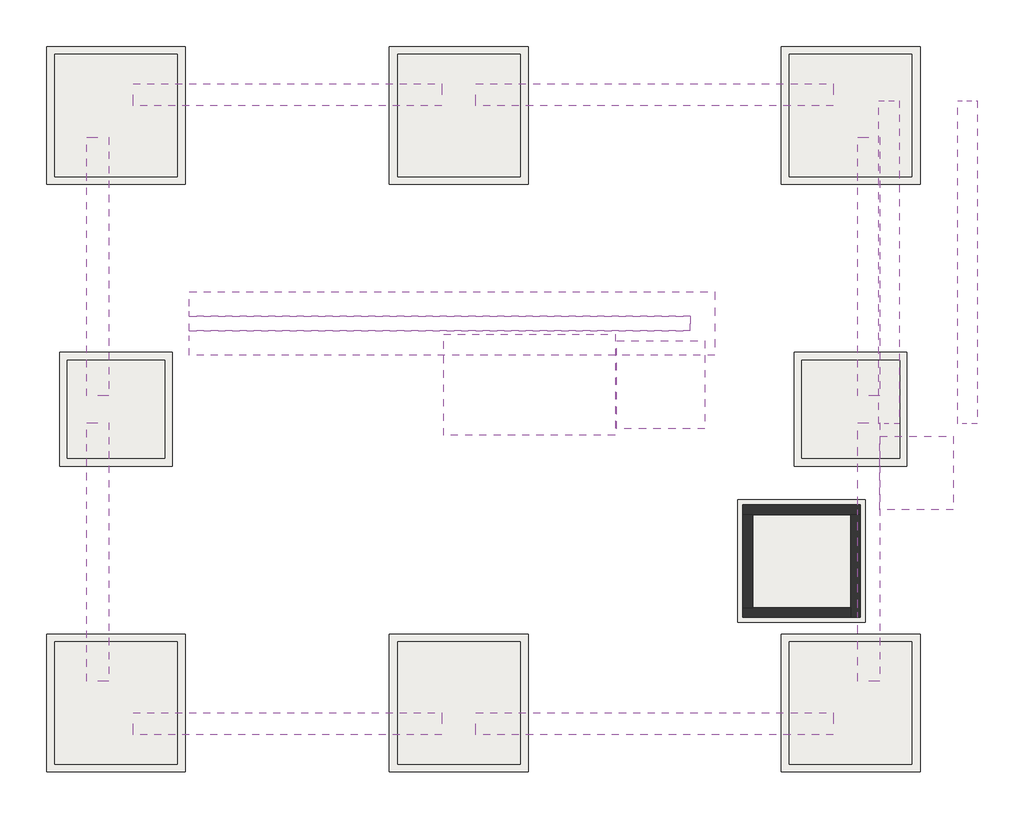
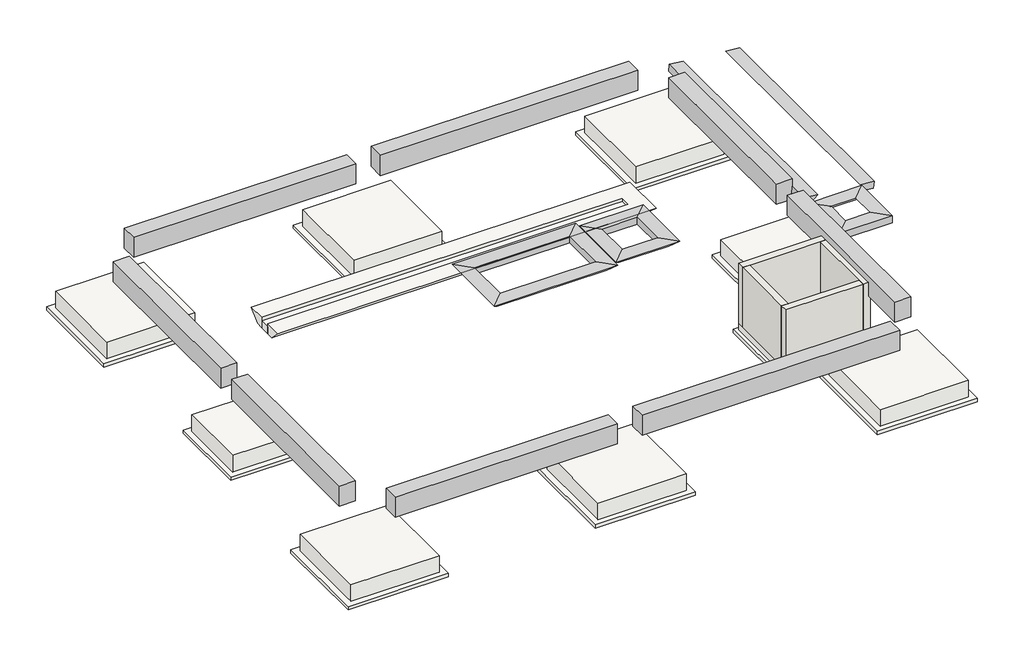
# One storey: 20 slabs, 7 beams, 5 proxies, 4 walls, 1 member.
# Revit data of these elements (continued)
# Project information (continued)
#     93-00152f0a\" ism_id=\"434ac00d-0b75-408a-b526-bf8655b26baf\" /><element revit_id=\"af7cfdda-f71a-4a09-bb03-63e0c16d5d93-00152f0c\" ism_id=\"5e4f7e2a-2154-47cc-93bc-24e7bd197632\" /><element revit_id=\"af7cfdda-f71a-4a09-bb03-63e0c16d5d93-00152f0e\" ism_id=\"f1998cd9-044c-4f7a-99e6-248bc5b45dba\" /><element revit_id=\"af7cfdda-f71a-4a09-bb03-63e0c16d5d93-00152f10\" ism_id=\"6ca0e144-6dd7-4824-b6a4-c3599ffcc64c\" /><element revit_id=\"af7cfdda-f71a-4a09-bb03-63e0c16d5d93-00152f12\" ism_id=\"173f1f07-ca52-4750-b7f6-1ef0180c36ba\" /><element revit_id=\"af7cfdda-f71a-4a09-bb03-63e0c16d5d93-00152f15\" ism_id=\"29a619d1-86ac-46c7-a220-2e78769b313e\" /><element revit_id=\"af7cfdda-f71a-4a09-bb03-63e0c16d5d93-00152f17\" ism_id=\"de21b25d-6b5e-4da6-89ee-8b671f1287ec\" /><element revit_id=\"af7cfdda-f71a-4a09-bb03-63e0c16d5d93-00152f19\" ism_id=\"70cdf538-eeaa-48c4-9315-181e56578638\" /><element revit_id=\"af7cfdda-f71a-4a09-bb03-63e0c16d5d93-00152f1b\" ism_id=\"49734cf8-a963-4163-b104-a25bff74fff0\" /><element revit_id=\"af7cfdda-f71a-4a09-bb03-63e0c16d5d93-00152f1d\" ism_id=\"a5a98e28-e98d-4759-bcab-d40632bfc19f\" /><element revit_id=\"af7cfdda-f71a-4a09-bb03-63e0c16d5d93-00152f1f\" ism_id=\"ab6af08f-90da-4d2f-a66a-db65621b8e94\" /><element revit_id=\"af7cfdda-f71a-4a09-bb03-63e0c16d5d93-00152f21\" ism_id=\"a65b64ab-134d-4223-82b7-5e66d90bc276\" /><element revit_id=\"af7cfdda-f71a-4a09-bb03-63e0c16d5d93-00152f23\" ism_id=\"6a1f317f-8940-4af8-9522-8e6c47c0c3a6\" /><element revit_id=\"af7cfdda-f71a-4a09-bb03-63e0c16d5d93-00152f25\" ism_id=\"880c6aab-7058-4382-9d83-6c759bdcf822\" /><element revit_id=\"af7cfdda-f71a-4a09-bb03-63e0c16d5d93-00152f27\" ism_id=\"555977b1-6494-4ee8-b235-8bae97762787\" /><element revit_id=\"af7cfdda-f71a-4a09-bb03-63e0c16d5d93-00152f29\" ism_id=\"66c9b467-8c65-4f1e-9542-95b43d793e9b\" /><element revit_id=\"af7cfdda-f71a-4a09-bb03-63e0c16d5d93-00152f2b\" ism_id=\"217a9ce2-64ab-4115-836e-06014fa1b21e\" /><element revit_id=\"af7cfdda-f71a-4a09-bb03-63e0c16d5d93-00152f2d\" ism_id=\"f7fc30da-832d-44e7-bab3-dd115d25639e\" /><element revit_id=\"af7cfdda-f71a-4a09-bb03-63e0c16d5d93-00152f2f\" ism_id=\"715eb46c-1b8d-4226-a7c6-6c6c165bf34d\" /><element revit_id=\"af7cfdda-f71a-4a09-bb03-63e0c16d5d93-00152f31\" ism_id=\"ef53c2b2-6fcf-42d2-96ea-f30a899bf64f\" /><element revit_id=\"af7cfdda-f71a-4a09-bb03-63e0c16d5d93-00152f34\" ism_id=\"1aefa093-18ee-4a97-8178-1b1fb4b7aceb\" /><element revit_id=\"af7cfdda-f71a-4a09-bb03-63e0c16d5d93-00152f38\" ism_id=\"262f02a9-64ca-487b-befd-4b58d44dffa7\" /><element revit_id=\"af7cfdda-f71a-4a09-bb03-63e0c16d5d93-00152f3b\" ism_id=\"6f2442a8-c4c0-4b53-9d7f-7059d6ededd2\" /><element revit_id=\"af7cfdda-f71a-4a09-bb03-63e0c16d5d93-00152f3e\" ism_id=\"dd838df4-69c7-406c-93e1-418c01f5734f\" /><element revit_id=\"af7cfdda-f71a-4a09-bb03-63e0c16d5d93-00152f40\" ism_id=\"9dec5077-28a7-4c32-95d2-08813de6a916\" /><element revit_id=\"af7cfdda-f71a-4a09-bb03-63e0c16d5d93-00152f42\" ism_id=\"9370ae5f-9277-4bb3-917b-cb3f318800a8\" /><element revit_id=\"af7cfdda-f71a-4a09-bb03-63e0c16d5d93-00152f44\" ism_id=\"0f3f2c81-58b4-4698-b1be-75061a4a2ae1\" /><element revit_id=\"af7cfdda-f71a-4a09-bb03-63e0c16d5d93-00152f46\" ism_id=\"95dca10f-6510-4ae7-a23e-7a1fd6939662\" /><element revit_id=\"af7cfdda-f71a-4a09-bb03-63e0c16d5d93-00152f49\" ism_id=\"83bad907-6a1c-4702-9990-a1a9c13d0160\" /><element revit_id=\"af7cfdda-f71a-4a09-bb03-63e0c16d5d93-00152f4d\" ism_id=\"7dba72dc-0de8-457c-8d3c-9c80941133ff\" /><element revit_id=\"af7cfdda-f71a-4a09-bb03-63e0c16d5d93-00152f51\" ism_id=\"a6cf3de2-949b-45b4-8029-061e06e5ab91\" /><element revit_id=\"af7cfdda-f71a-4a09-bb03-63e0c16d5d93-00152f54\" ism_id=\"77af5754-dd62-4c90-accb-d0b9405b5baf\" /><element revit_id=\"af7cfdda-f71a-4a09-bb03-63e0c16d5d93-00152f56\" ism_id=\"6461cb37-823d-49bb-bea2-3dbd4db85a81\" /><element revit_id=\"af7cfdda-f71a-4a09-bb03-63e0c16d5d93-00152f59\" ism_id=\"e2f2909f-27bc-426e-b2db-27b1217d3560\" /><element revit_id=\"af7cfdda-f71a-4a09-bb03-63e0c16d5d93-00152f5b\" ism_id=\"46c410de-fc65-4593-ae24-da1a154b45fb\" /><element revit_id=\"af7cfdda-f71a-4a09-bb03-63e0c16d5d93-00152f5d\" ism_id=\"d7d73cf7-a31f-421c-bc39-3ba338a334b1\" /><element revit_id=\"af7cfdda-f71a-4a09-bb03-63e0c16d5d93-00152f61\" ism_id=\"6bd81f7b-5fd8-4f19-ad3a-4e009274854c\" /><element revit_id=\"af7cfdda-f71a-4a09-bb03-63e0c16d5d93-00152f64\" ism_id=\"f25b9af0-504f-4aaf-a359-d2bc9d32b683\" /><element revit_id=\"af7cfdda-f71a-4a09-bb03-63e0c16d5d93-00152f66\" ism_id=\"f143dcd3-1cc7-47ae-b4ed-c960a7d1349c\" /><element revit_id=\"af7cfdda-f71a-4a09-bb03-63e0c16d5d93-00152f68\" ism_id=\"296e8d7f-a89b-405a-b793-fc1ea4b11be5\" /><element revit_id=\"af7cfdda-f71a-4a09-bb03-63e0c16d5d93-00152f6b\" ism_id=\"48b24488-3184-439c-b285-73e81edfef17\" /><element revit_id=\"af7cfdda-f71a-4a09-bb03-63e0c16d5d93-00152f6e\" ism_id=\"0db0ccd4-631c-4972-aad8-2fd483c55629\" /><element revit_id=\"af7cfdda-f71a-4a09-bb03-63e0c16d5d93-00152f71\" ism_id=\"ee51bd40-01d8-4a48-92c6-90509a96cad2\" /><element revit_id=\"af7cfdda-f71a-4a09-bb03-63e0c16d5d93-00152f73\" ism_id=\"e5c66ce6-ca9d-4591-9d75-5348307a88bc\" /><element revit_id=\"af7cfdda-f71a-4a09-bb03-63e0c16d5d93-00152f75\" ism_id=\"892d82ae-6f73-4af5-8575-78955f2b6c3b\" /><element revit_id=\"af7cfdda-f71a-4a09-bb03-63e0c16d5d93-00152f78\" ism_id=\"cb5b2a2e-5551-4b87-9d0b-6382c09e6ce2\" /><element revit_id=\"af7cfdda-f71a-4a09-bb03-63e0c16d5d93-00152f7c\" ism_id=\"1177c4ab-d04b-426b-80ba-afa1f1403e20\" /><element revit_id=\"af7cfdda-f71a-4a09-bb03-63e0c16d5d93-00152f7f\" ism_id=\"235d8a18-f10a-44ad-8945-ebb2f02646fa\" /><element revit_id=\"af7cfdda-f71a-4a09-bb03-63e0c16d5d93-00152f83\" ism_id=\"6127db9d-7d4b-44c8-806c-e4f7d278db0c\" /><element revit_id=\"af7cfdda-f71a-4a09-bb03-63e0c16d5d93-00152f86\" ism_id=\"85d79da8-d317-4e5b-88a2-88d20cb73d7d\" /><element revit_id=\"af7cfdda-f71a-4a09-bb03-63e0c16d5d93-00152f89\" ism_id=\"f4105a19-7c5e-4970-9446-50e578b67af2\" /><element revit_id=\"af7cfdda-f71a-4a09-bb03-63e0c16d5d93-00152f8b\" ism_id=\"ab299061-87b1-4edc-8a5c-c55542368f39\" /><element revit_id=\"af7cfdda-f71a-4a09-bb03-63e0c16d5d93-00152f8d\" ism_id=\"43097401-25be-48d4-a7ba-f3c37c1b84e9\" /><element revit_id=\"af7cfdda-f71a-4a09-bb03-63e0c16d5d93-00152f8f\" ism_id=\"fd9214b7-59e9-4736-b544-a37d4c180e24\" /><element revit_id=\"af7cfdda-f71a-4a09-bb03-63e0c16d5d93-00152f91\" ism_id=\"b83d1d95-2d97-4532-8a94-368577601c17\" /><element revit_id=\"af7cfdda-f71a-4a09-bb03-63e0c16d5d93-00152f94\" ism_id=\"9bd5e620-e2eb-4ede-9a8b-b0183e171248\" /><element revit_id=\"af7cfdda-f71a-4a09-bb03-63e0c16d5d93-00152f97\" ism_id=\"d6f9d903-1605-43dc-872c-2f9de6642af6\" /><element revit_id=\"af7cfdda-f71a-4a09-bb03-63e0c16d5d93-00152f99\" ism_id=\"7c236b12-3da8-4ae0-bc99-2aa089118476\" /><element revit_id=\"af7cfdda-f71a-4a09-bb03-63e0c16d5d93-00152f9b\" ism_id=\"2b88d03d-aeef-4f51-b98c-562513d6f6da\" /><element revit_id=\"af7cfdda-f71a-4a09-bb03-63e0c16d5d93-00152f9d\" ism_id=\"6639b07f-6759-4580-bc0a-91cdbc82216d\" /><element revit_id=\"af7cfdda-f71a-4a09-bb03-63e0c16d5d93-00152f9f\" ism_id=\"d17e7cf5-d760-4c38-8bb0-8a57fe45e3ad\" /><element revit_id=\"af7cfdda-f71a-4a09-bb03-63e0c16d5d93-00152fa2\" ism_id=\"6dbdf2a2-22ac-4132-a9ae-8992fe15b0d7\" /><element revit_id=\"af7cfdda-f71a-4a09-bb03-63e0c16d5d93-00152fa4\" ism_id=\"663381be-9f3f-499f-b7c1-64170401ecb3\" /><element revit_id=\"af7cfdda-f71a-4a09-bb03-63e0c16d5d93-00152fa6\" ism_id=\"5ba3ff14-3d24-47a8-9418-aecce16bd943\" /><element revit_id=\"af7cfdda-f71a-4a09-bb03-63e0c16d5d93-00152fa8\" ism_id=\"8f845e6a-1432-4c61-8362-e12c105320fb\" /><element revit_id=\"af7cfdda-f71a-4a09-bb03-63e0c16d5d93-00152faa\" ism_id=\"263897bf-02c2-4ed7-8e3f-2020d545125e\" /><element revit_id=\"af7cfdda-f71a-4a09-bb03-63e0c16d5d93-00152fac\" ism_id=\"f1241312-d990-4c87-92ff-afc1975a3d67\" /><element revit_id=\"af7cfdda-f71a-4a09-bb03-63e0c16d5d93-00152fae\" ism_id=\"5740cb23-0cbc-47ce-acea-31b5a043bf0c\" /><element revit_id=\"af7cfdda-f71a-4a09-bb03-63e0c16d5d93-00152fb0\" ism_id=\"7aeaeafb-f9bc-4bee-b237-caade22069b8\" /><element revit_id=\"af7cfdda-f71a-4a09-bb03-63e0c16d5d93-00152fb3\" ism_id=\"90084dda-e197-4e46-8e5b-4f629a594830\" /><element revit_id=\"af7cfdda-f71a-4a09-bb03-63e0c16d5d93-00152fb5\" ism_id=\"2c392f12-2b50-4bd2-8c41-ef64640e587b\" /><element revit_id=\"af7cfdda-f71a-4a09-bb03-63e0c16d5d93-00152fb7\" ism_id=\"d25284c0-6931-4cbb-8ed3-63397f6a5616\" /><element revit_id=\"af7cfdda-f71a-4a09-bb03-63e0c16d5d93-00152fb9\" ism_id=\"32799d39-e9bc-468c-ac64-a3f2c8e075af\" /><element revit_id=\"af7cfdda-f71a-4a09-bb03-63e0c16d5d93-00152fbb\" ism_id=\"61a092b8-d924-4e61-a1ef-adc051541aaf\" /><element revit_id=\"af7cfdda-f71a-4a09-bb03-63e0c16d5d93-00152fbe\" ism_id=\"ae89ad42-0006-42ee-9328-01a896002b7a\" /><element revit_id=\"af7cfdda-f71a-4a09-bb03-63e0c16d5d93-00152fc0\" ism_id=\"7b4d47fd-5fcd-4692-9b39-36bb95372647\" /><element revit_id=\"af7cfdda-f71a-4a09-bb03-63e0c16d5d93-00152fc2\" ism_id=\"150f022d-eb78-47d8-8d70-c7ea5433f366\" /><element revit_id=\"af7cfdda-f71a-4a09-bb03-63e0c16d5d93-00152fc4\" ism_id=\"6780451e-52c6-4962-8bb4-f1fd57bf7865\" /><element revit_id=\"af7cfdda-f71a-4a09-bb03-63e0c16d5d93-00152fc6\" ism_id=\"b3896748-2d7c-424b-ae81-8b769d840fbc\" /><element revit_id=\"af7cfdda-f71a-4a09-bb03-63e0c16d5d93-00152fc9\" ism_id=\"0c64c745-ce95-4f37-8a9d-d07fd5d17ecb\" /><element revit_id=\"af7cfdda-f71a-4a09-bb03-63e0c16d5d93-00152fcc\" ism_id=\"dc23390d-d501-4d7e-9369-f7793a7306a7\" /><element revit_id=\"af7cfdda-f71a-4a09-bb03-63e0c16d5d93-00152fcf\" ism_id=\"a2d2dfc7-08e7-459b-9de9-2d46c1b9d65d\" /><element revit_id=\"af7cfdda-f71a-4a09-bb03-63e0c16d5d93-00152fd2\" ism_id=\"0357c393-c221-46b8-a525-7eece05024d5\" /><element revit_id=\"af7cfdda-f71a-4a09-bb03-63e0c16d5d93-00152fd4\" ism_id=\"7514ec1a-cc54-428f-bbfe-53465c7b9971\" /><element revit_id=\"af7cfdda-f71a-4a09-bb03-63e0c16d5d93-00152fd7\" ism_id=\"f5e61f1a-565d-4eed-b8cc-74798bf49f83\" /><element revit_id=\"af7cfdda-f71a-4a09-bb03-63e0c16d5d93-00152fd9\" ism_id=\"7d7031a0-6061-49e6-8bb3-df1503ddb602\" /><element revit_id=\"af7cfdda-f71a-4a09-bb03-63e0c16d5d93-00152fdb\" ism_id=\"0d733cbc-e2dd-44ec-a5f3-da43d2d7ec46\" /><element revit_id=\"af7cfdda-f71a-4a09-bb03-63e0c16d5d93-00152fdd\" ism_id=\"21cbc8e9-c640-4a2e-8958-1d3b7a784879\" /><element revit_id=\"af7cfdda-f71a-4a09-bb03-63e0c16d5d93-00152fdf\" ism_id=\"fac86bbb-1d81-4320-81cd-30997be31eb4\" /><element revit_id=\"af7cfdda-f71a-4a09-bb03-63e0c16d5d93-00152fe1\" ism_id=\"ebc7c696-170e-4ba4-8599-103279d331b8\" /><element revit_id=\"af7cfdda-f71a-4a09-bb03-63e0c16d5d93-00152fe3\" ism_id=\"91dec439-7fd8-4259-bbce-df46237765e2\" /><element revit_id=\"af7cfdda-f71a-4a09-bb03-63e0c16d5d93-00152fe5\" ism_id=\"6227503a-c521-4b5a-b5c3-b9e2ea2b5c81\" /><element revit_id=\"af7cfdda-f71a-4a09-bb03-63e0c16d5d93-00152fe7\" ism_id=\"e6e91966-53ab-4536-84a0-3f6e5a22fbeb\" /><element revit_id=\"af7cfdda-f71a-4a09-bb03-63e0c16d5d93-00152fe9\" ism_id=\"fb3387b3-301c-40a5-8217-97be67c50843\" /><element revit_id=\"af7cfdda-f71a-4a09-bb03-63e0c16d5d93-00152feb\" ism_id=\"37825fc8-0fe2-440e-933a-1453c922c9d9\" /><element revit_id=\"af7cfdda-f71a-4a09-bb03-63e0c16d5d93-00152fed\" ism_id=\"06b175df-5526-4920-a3d6-7f2ff872756e\" /><element revit_id=\"af7cfdda-f71a-4a09-bb03-63e0c16d5d93-00152fef\" ism_id=\"a8fbce7a-6989-46e5-9bc5-c497d4a295c9\" /><element revit_id=\"af7cfdda-f71a-4a09-bb03-63e0c16d5d93-00152ff1\" ism_id=\"cf8ccf89-d0da-4b4e-93d8-85d639853d5e\" /><element revit_id=\"af7cfdda-f71a-4a09-bb03-63e0c16d5d93-00152ff3\" ism_id=\"1b85e87c-6c2a-4057-8491-40e4237cd0e6\" /><element revit_id=\"af7cfdda-f71a-4a09-bb03-63e0c16d5d93-00152ff5\" ism_id=\"69be497f-343c-4d38-9ea0-e959474332f8\" /><element revit_id=\"af7cfdda-f71a-4a09-bb03-63e0c16d5d93-00152ff7\" ism_id=\"72738956-f87a-41b4-a019-35adc3bff764\" /><element revit_id=\"af7cfdda-f71a-4a09-bb03-63e0c16d5d93-00152ff9\" ism_id=\"f127b15c-142d-4b57-83a6-5b76ac4cde6e\" /><element revit_id=
#     \"af7cfdda-f71a-4a09-bb03-63e0c16d5d93-00152ffb\" ism_id=\"3a38a709-bfa8-404e-b889-5af5e78ea0bf\" /><element revit_id=\"af7cfdda-f71a-4a09-bb03-63e0c16d5d93-00152ffe\" ism_id=\"bebf0363-7e59-4a43-8f5b-502fcc4a338d\" /><element revit_id=\"af7cfdda-f71a-4a09-bb03-63e0c16d5d93-00153000\" ism_id=\"157fe154-0d28-4e8c-a143-e2896867fd28\" /><element revit_id=\"af7cfdda-f71a-4a09-bb03-63e0c16d5d93-00153002\" ism_id=\"1bf52bf8-7327-4d55-b5cd-bf7c9bf89688\" /><element revit_id=\"af7cfdda-f71a-4a09-bb03-63e0c16d5d93-00153005\" ism_id=\"7a0025bf-d54b-4614-9002-7bd4a82da90e\" /><element revit_id=\"af7cfdda-f71a-4a09-bb03-63e0c16d5d93-00153008\" ism_id=\"cad53638-8c8f-4a89-ab6f-d8a32131833b\" /><element revit_id=\"af7cfdda-f71a-4a09-bb03-63e0c16d5d93-0015300a\" ism_id=\"05672ccd-1a96-434c-8da1-7a706b3561f7\" /><element revit_id=\"af7cfdda-f71a-4a09-bb03-63e0c16d5d93-0015300c\" ism_id=\"bb809016-b2bb-4157-847e-1cca3692ba19\" /><element revit_id=\"af7cfdda-f71a-4a09-bb03-63e0c16d5d93-0015300f\" ism_id=\"720ed192-8aa7-46fd-9f7a-15d64351767c\" /><element revit_id=\"af7cfdda-f71a-4a09-bb03-63e0c16d5d93-00153011\" ism_id=\"9a47cdb9-976d-41f3-a5c3-5a7516a7763c\" /><element revit_id=\"af7cfdda-f71a-4a09-bb03-63e0c16d5d93-00153013\" ism_id=\"aba01787-c82b-453e-8db2-70277a34d5ad\" /><element revit_id=\"af7cfdda-f71a-4a09-bb03-63e0c16d5d93-00153015\" ism_id=\"f6b882e3-d64a-44b1-878c-9c00ee1fde86\" /><element revit_id=\"af7cfdda-f71a-4a09-bb03-63e0c16d5d93-00153017\" ism_id=\"95108815-490a-427a-aec1-8fcefc57c858\" /><element revit_id=\"af7cfdda-f71a-4a09-bb03-63e0c16d5d93-00153019\" ism_id=\"8fe55cf1-56b4-4a62-948a-d7f0c95bd04b\" /><element revit_id=\"af7cfdda-f71a-4a09-bb03-63e0c16d5d93-0015301b\" ism_id=\"b889bf8b-3bdd-410a-b11b-9ca69449d470\" /><element revit_id=\"af7cfdda-f71a-4a09-bb03-63e0c16d5d93-0015301d\" ism_id=\"ef8604de-de5b-45ec-9158-0b702e6ef713\" /><element revit_id=\"af7cfdda-f71a-4a09-bb03-63e0c16d5d93-0015301f\" ism_id=\"40ee286a-4bc9-4d4f-ba6d-fe1ac9da03cf\" /><element revit_id=\"af7cfdda-f71a-4a09-bb03-63e0c16d5d93-00153021\" ism_id=\"cc903f39-6bdf-4081-a56c-883169221735\" /><element revit_id=\"af7cfdda-f71a-4a09-bb03-63e0c16d5d93-00153023\" ism_id=\"0af04955-dcb6-4295-b3d4-7c432a233062\" /><element revit_id=\"af7cfdda-f71a-4a09-bb03-63e0c16d5d93-00153025\" ism_id=\"75a51549-6a04-4399-b818-f170a8c10286\" /><element revit_id=\"af7cfdda-f71a-4a09-bb03-63e0c16d5d93-00153027\" ism_id=\"7e183794-5c66-46bc-97f5-2df209b3286d\" /><element revit_id=\"af7cfdda-f71a-4a09-bb03-63e0c16d5d93-00153029\" ism_id=\"ed4a7448-29b0-44e3-8b6f-7310f83440ab\" /><element revit_id=\"af7cfdda-f71a-4a09-bb03-63e0c16d5d93-0015302b\" ism_id=\"fdb5eb17-b94e-40c1-b703-3ecb5e4efee4\" /><element revit_id=\"af7cfdda-f71a-4a09-bb03-63e0c16d5d93-0015302d\" ism_id=\"779397c1-65b7-447f-a72e-2a09308021ea\" /><element revit_id=\"af7cfdda-f71a-4a09-bb03-63e0c16d5d93-0015302f\" ism_id=\"7b409707-86c5-44e2-919e-92ad5bb9eb8b\" /><element revit_id=\"af7cfdda-f71a-4a09-bb03-63e0c16d5d93-00153031\" ism_id=\"d337c78b-590d-406c-bf20-6a3558821db1\" /><element revit_id=\"af7cfdda-f71a-4a09-bb03-63e0c16d5d93-00153033\" ism_id=\"c27f5f6d-8445-4415-853d-d316787bea6e\" /><element revit_id=\"af7cfdda-f71a-4a09-bb03-63e0c16d5d93-00153035\" ism_id=\"76036a55-3bab-417a-ba41-ec1335e2e2a7\" /><element revit_id=\"af7cfdda-f71a-4a09-bb03-63e0c16d5d93-00153037\" ism_id=\"24be638c-ff89-4616-8974-5b79c81e6e56\" /><element revit_id=\"af7cfdda-f71a-4a09-bb03-63e0c16d5d93-00153039\" ism_id=\"015f9f2c-2353-4795-b891-e4ee986f25f7\" /><element revit_id=\"af7cfdda-f71a-4a09-bb03-63e0c16d5d93-0015303b\" ism_id=\"91f8ddfb-c5b9-4f33-b141-a6edfbccf098\" /><element revit_id=\"af7cfdda-f71a-4a09-bb03-63e0c16d5d93-0015303d\" ism_id=\"78540364-1ba5-4f0c-95fb-ba8631e32695\" /><element revit_id=\"af7cfdda-f71a-4a09-bb03-63e0c16d5d93-0015303f\" ism_id=\"9d53e406-367b-4e3e-b5e8-d421731e1aab\" /><element revit_id=\"af7cfdda-f71a-4a09-bb03-63e0c16d5d93-00153041\" ism_id=\"24aa6051-1a20-4f08-8962-6f6f9ff4dc98\" /><element revit_id=\"af7cfdda-f71a-4a09-bb03-63e0c16d5d93-00153043\" ism_id=\"572a4144-5250-4962-a1b9-09502cda2774\" /><element revit_id=\"af7cfdda-f71a-4a09-bb03-63e0c16d5d93-00153045\" ism_id=\"1f486980-0be9-4aad-b32e-0608218bf68e\" /><element revit_id=\"af7cfdda-f71a-4a09-bb03-63e0c16d5d93-00153047\" ism_id=\"588ed856-d113-4521-b97c-a4d7ac7ba406\" /><element revit_id=\"af7cfdda-f71a-4a09-bb03-63e0c16d5d93-00153049\" ism_id=\"741942b7-995d-48cb-8401-4faec8ef8d15\" /><element revit_id=\"af7cfdda-f71a-4a09-bb03-63e0c16d5d93-0015304b\" ism_id=\"85254c30-08c9-46e3-acd6-6b5131f485ce\" /><element revit_id=\"af7cfdda-f71a-4a09-bb03-63e0c16d5d93-0015304e\" ism_id=\"2d57d6c0-67d8-48bd-b16f-8ef7edb485b1\" /><element revit_id=\"af7cfdda-f71a-4a09-bb03-63e0c16d5d93-00153050\" ism_id=\"57b4caff-473e-4ebc-b42c-d73ce4ca67d8\" /><element revit_id=\"af7cfdda-f71a-4a09-bb03-63e0c16d5d93-00153052\" ism_id=\"1adae240-a487-478c-a898-61bee40e7415\" /><element revit_id=\"af7cfdda-f71a-4a09-bb03-63e0c16d5d93-00153054\" ism_id=\"62613b5f-092e-4f63-86ac-d3e070a85bc5\" /><element revit_id=\"af7cfdda-f71a-4a09-bb03-63e0c16d5d93-00153056\" ism_id=\"6aecb1de-b991-4eed-80ad-e1b9ccc03a87\" /><element revit_id=\"af7cfdda-f71a-4a09-bb03-63e0c16d5d93-00153058\" ism_id=\"ecab5d8d-84d0-44a4-9549-bca959ac514b\" /><element revit_id=\"af7cfdda-f71a-4a09-bb03-63e0c16d5d93-0015305a\" ism_id=\"589f44ad-061b-46bc-91bd-bf9b1e708415\" /><element revit_id=\"af7cfdda-f71a-4a09-bb03-63e0c16d5d93-0015305c\" ism_id=\"bfa24af8-499f-45ff-9e9d-d5cc0761fed6\" /><element revit_id=\"af7cfdda-f71a-4a09-bb03-63e0c16d5d93-0015305e\" ism_id=\"8114f473-ca73-4cc8-b3e2-979f07368f66\" /><element revit_id=\"af7cfdda-f71a-4a09-bb03-63e0c16d5d93-00153060\" ism_id=\"4dde7439-2ac9-412f-a5f5-e9fd0f294ec8\" /><element revit_id=\"af7cfdda-f71a-4a09-bb03-63e0c16d5d93-00153062\" ism_id=\"661cc7d8-fd9c-4505-b43e-241bfd24b2d0\" /><element revit_id=\"af7cfdda-f71a-4a09-bb03-63e0c16d5d93-00153064\" ism_id=\"1e7f186f-1b55-4d4c-bf9f-18595049605e\" /><element revit_id=\"af7cfdda-f71a-4a09-bb03-63e0c16d5d93-00153066\" ism_id=\"ee968183-c9c6-4eab-86cf-0eda12de724b\" /><element revit_id=\"af7cfdda-f71a-4a09-bb03-63e0c16d5d93-00153068\" ism_id=\"5de1f319-cdd1-4b9a-8f8e-b86394effa22\" /><element revit_id=\"af7cfdda-f71a-4a09-bb03-63e0c16d5d93-0015306a\" ism_id=\"fa557a6c-2e39-4481-9eb5-5ede8fd31c49\" /><element revit_id=\"af7cfdda-f71a-4a09-bb03-63e0c16d5d93-0015306c\" ism_id=\"b2710e8e-0f5f-4e74-a366-aef04da22cd3\" /><element revit_id=\"af7cfdda-f71a-4a09-bb03-63e0c16d5d93-0015306e\" ism_id=\"5633c3b7-f903-46ee-b126-8a20a9a62c90\" /><element revit_id=\"af7cfdda-f71a-4a09-bb03-63e0c16d5d93-00153070\" ism_id=\"62796ef8-c4bb-4b9f-bd14-cc7392046eb4\" /><element revit_id=\"af7cfdda-f71a-4a09-bb03-63e0c16d5d93-00153072\" ism_id=\"db898ada-150e-4ff5-a9f8-16e27b46b754\" /><element revit_id=\"af7cfdda-f71a-4a09-bb03-63e0c16d5d93-00153075\" ism_id=\"d3965d2d-e119-4f6b-af8d-52c8a5397d36\" /><element revit_id=\"af7cfdda-f71a-4a09-bb03-63e0c16d5d93-00153077\" ism_id=\"063574e4-6319-4ba7-8e34-1638a1357d5f\" /><element revit_id=\"af7cfdda-f71a-4a09-bb03-63e0c16d5d93-00153079\" ism_id=\"6de69805-8980-44f0-9316-6d50d1b47cbb\" /><element revit_id=\"af7cfdda-f71a-4a09-bb03-63e0c16d5d93-0015307b\" ism_id=\"e5f77c5b-4806-4993-8875-6149db708e42\" /><element revit_id=\"af7cfdda-f71a-4a09-bb03-63e0c16d5d93-0015307d\" ism_id=\"a13071c9-c086-4896-95a6-a015bc531f25\" /><element revit_id=\"af7cfdda-f71a-4a09-bb03-63e0c16d5d93-0015307f\" ism_id=\"c9d216f9-adca-4752-b8c1-d779727505dd\" /><element revit_id=\"af7cfdda-f71a-4a09-bb03-63e0c16d5d93-00153081\" ism_id=\"5b167621-3850-4169-8bee-1e0420bf6050\" /><element revit_id=\"af7cfdda-f71a-4a09-bb03-63e0c16d5d93-00153083\" ism_id=\"09cf76ae-a083-4203-a622-7e9424374f66\" /><element revit_id=\"af7cfdda-f71a-4a09-bb03-63e0c16d5d93-00153085\" ism_id=\"14063b50-058d-464a-aa08-369865983eeb\" /><element revit_id=\"af7cfdda-f71a-4a09-bb03-63e0c16d5d93-00153087\" ism_id=\"add5837f-63be-4349-b708-9f4051059e25\" /><element revit_id=\"af7cfdda-f71a-4a09-bb03-63e0c16d5d93-00153089\" ism_id=\"b4c60bd3-61cb-423f-916a-fa2b71585228\" /><element revit_id=\"af7cfdda-f71a-4a09-bb03-63e0c16d5d93-0015308b\" ism_id=\"6251d90e-381f-4771-818c-f7465ae91864\" /><element revit_id=\"af7cfdda-f71a-4a09-bb03-63e0c16d5d93-0015308d\" ism_id=\"7693be9d-48ca-4005-bed4-90e9c08d3a38\" /><element revit_id=\"af7cfdda-f71a-4a09-bb03-63e0c16d5d93-0015308f\" ism_id=\"a6a39ca9-cd56-43ba-bfe8-2cf3b78878cc\" /><element revit_id=\"af7cfdda-f71a-4a09-bb03-63e0c16d5d93-00153091\" ism_id=\"1a3956c4-77bb-4ccc-a12d-c3514cf365d4\" /><element revit_id=\"af7cfdda-f71a-4a09-bb03-63e0c16d5d93-00153093\" ism_id=\"2ffa7a89-8ee9-470a-b3d8-7c27f566e226\" /><element revit_id=\"af7cfdda-f71a-4a09-bb03-63e0c16d5d93-00153095\" ism_id=\"e865b460-944f-4057-a6e8-4e39cb88d97d\" /><element revit_id=\"af7cfdda-f71a-4a09-bb03-63e0c16d5d93-00153097\" ism_id=\"69410bb9-8440-4a88-9151-b5459095fe2e\" /><element revit_id=\"af7cfdda-f71a-4a09-bb03-63e0c16d5d93-00153099\" ism_id=\"1efae87b-0246-432c-a428-82c87fb3929c\" /><element revit_id=\"af7cfdda-f71a-4a09-bb03-63e0c16d5d93-0015309b\" ism_id=\"e1d5fb57-3b5d-4a32-bccb-cea278671f2f\" /><element revit_id=\"af7cfdda-f71a-4a09-bb03-63e0c16d5d93-0015309d\" ism_id=\"c74a7061-f4b2-41b5-b3ff-caf6cf9dfffd\" /><element revit_id=\"af7cfdda-f71a-4a09-bb03-63e0c16d5d93-0015309f\" ism_id=\"aa777ec3-1257-49eb-b597-fbab7bda8b11\" /><element revit_id=\"af7cfdda-f71a-4a09-bb03-63e0c16d5d93-001530a1\" ism_id=\"7420a67b-bb48-477d-823a-c473ce92c083\" /><element revit_id=\"af7cfdda-f71a-4a09-bb03-63e0c16d5d93-001530a3\" ism_id=\"1ee9340a-8778-4cd6-be2d-57fb5fe16e45\" /><element revit_id=\"af7cfdda-f71a-4a09-bb03-63e0c16d5d93-001530a5\" ism_id=\"3216ac21-29b0-45a7-a070-99a114df4980\" /><element revit_id=\"af7cfdda-f71a-4a09-bb03-63e0c16d5d93-001530a7\" ism_id=\"dce9c5c3-a57a-4091-8398-cace2e63f290\" /><element revit_id=\"af7cfdda-f71a-4a09-bb03-63e0c16d5d93-001530a9\" ism_id=\"dcadcd2e-1b12-41e7-a9d5-5d99303c7e51\" /><element revit_id=\"af7cfdda-f71a-4a09-bb03-63e0c16d5d93-001530ab\" ism_id=\"ed4bf433-a5ea-40d4-8551-b735160eed03\" /><element revit_id=\"af7cfdda-f71a-4a09-bb03-63e0c16d5d93-001530ad\" ism_id=\"2cd91197-39b9-4301-8775-b1530f8812f8\" /><element revit_id=\"af7cfdda-f71a-4a09-bb03-63e0c16d5d93-001530af\" ism_id=\"53460b48-5382-4fff-98f2-ab500700bbca\" /><element revit_id=\"af7cfdda-f71a-4a09-bb03-63e0c16d5d93-001530b1\" ism_id=\"0d733cb9-b11e-45a1-89e1-53989b2ba4d5\" /><element revit_id=\"af7cfdda-f71a-4a09-bb03-63e0c16d5d93-001530b3\" ism_id=\"9b6990cb-bf48-452d-9572-952a8acd923b\" /><element revit_id=\"af7cfdda-f71a-4a09-bb03-63e0c16d5d93-001530b5\" ism_id=\"edb53df5-f0f8-45af-a38d-8c910b94c4aa\" /><element revit_id=\"af7cfdda-f71a-4a09-bb03-63e0c16d5d93-001530b7\" ism_id=\"a42a99cd-d791-460b-b7db-769eef45d4ee\" /><element revit_id=\"af7cfdda-f71a-4a09-bb03-63e0c16d5d93-001530b9\" ism_id=\"473eafff-0971-4b1a-8b61-a7662a5d0782\" /><element revit_id=\"af7cfdda-f71a-4a09-bb03-63e0c16d5d93-001530bb\" ism_id=\"b801d819-54a6-4fd3-91e7-5d49978bee50\" /><element revit_id=\"af7cfdda-f71a-4a09-bb03-63e0c16d5d93-001530bd\" ism_id=\"aa72d39c-13a9-4733-9528-98e90ae2a493\" /><element revit_id=\"af7cfdda-f71a-4a09-bb03-63e0c16d5d93-001530c0\" ism_id=\"e50950ab-c982-40e9-a130-a8fe9c5071aa\" /><element revit_id=\"af7cfdda-f71a-4a09-bb03-63e0c16d5d93-001530c3\" ism_id=\"caa8c896-9dda-4bb9-b942-fab7d7988525\" /><element revit_id=\"af7cfdda-f71a-4a09-bb03-63e0c16d5d93-001530c5\" ism_id=\"45f4fe9a-436c-4b4d-a48d-573edf59a390\" /><element revit_id=\"af7cfdda-f71a-4a09-bb03-63e0c16d5d93-001530c7\" ism_id=\"eb513efb-1058-4d3f-8f19-56219176a71a\" /><element revit_id=\"af7cfdda-f71a-4a09-bb03-63e0c16d5d93-001530c9\" ism_id=\"537abf12-3423-4f70-8613-a81d434152a6\" /><element revit_id=\"af7cfdda-f71a-4a09-bb03-63e0c16d5d93-001530cb\" ism_id=\"683f9f6d-960e-4ae9-ad7f-39eee39c3d47\" /><element revit_id=\"af7cfdda-f71a-4a09-bb03-63e0c16d5d93-001530cd\" ism_id=\"2ceed54c-aecf-4b75-a53e
#     -cfd758078946\" /><element revit_id=\"af7cfdda-f71a-4a09-bb03-63e0c16d5d93-001530cf\" ism_id=\"46a5ded9-4fed-43a0-a06e-bb0fce603002\" /><element revit_id=\"af7cfdda-f71a-4a09-bb03-63e0c16d5d93-001530d1\" ism_id=\"62d05a0c-55f2-4c29-a355-b77f91c84c50\" /><element revit_id=\"af7cfdda-f71a-4a09-bb03-63e0c16d5d93-001530d3\" ism_id=\"eac0c420-7041-45a3-ad98-0cab4f5d8155\" /><element revit_id=\"af7cfdda-f71a-4a09-bb03-63e0c16d5d93-001530d5\" ism_id=\"9f5beb51-429a-4c7b-aa2e-ad2efe601ed6\" /><element revit_id=\"af7cfdda-f71a-4a09-bb03-63e0c16d5d93-001530d7\" ism_id=\"4613af3e-a189-4781-a937-106d789655c9\" /><element revit_id=\"af7cfdda-f71a-4a09-bb03-63e0c16d5d93-001530d9\" ism_id=\"71402e21-51c1-43b7-b8cc-75d2aba247eb\" /><element revit_id=\"af7cfdda-f71a-4a09-bb03-63e0c16d5d93-001530db\" ism_id=\"89101b83-9b84-4f11-b026-90cd564a3900\" /><element revit_id=\"af7cfdda-f71a-4a09-bb03-63e0c16d5d93-001530dd\" ism_id=\"37670781-ce23-4ce1-992b-7a400613c37b\" /><element revit_id=\"af7cfdda-f71a-4a09-bb03-63e0c16d5d93-001530df\" ism_id=\"2316856d-18eb-466b-8ab8-114816378db0\" /><element revit_id=\"af7cfdda-f71a-4a09-bb03-63e0c16d5d93-001530e2\" ism_id=\"da4f1597-5b5a-43a6-aa94-e478ffd6cfc7\" /><element revit_id=\"af7cfdda-f71a-4a09-bb03-63e0c16d5d93-001530e5\" ism_id=\"60805764-efb2-4434-8d81-aed3c3ed3c1b\" /><element revit_id=\"af7cfdda-f71a-4a09-bb03-63e0c16d5d93-001530e8\" ism_id=\"34e34ebb-6481-4bfb-b3d0-cb52295ff652\" /><element revit_id=\"af7cfdda-f71a-4a09-bb03-63e0c16d5d93-001530eb\" ism_id=\"dd5c4d73-1406-4c40-a955-5f9c52d01161\" /><element revit_id=\"af7cfdda-f71a-4a09-bb03-63e0c16d5d93-001530ed\" ism_id=\"cf8abc6b-638f-4bd5-8b66-615be032e220\" /><element revit_id=\"af7cfdda-f71a-4a09-bb03-63e0c16d5d93-001530f0\" ism_id=\"56ce8857-0c24-48d5-82f2-459e263998e2\" /><element revit_id=\"af7cfdda-f71a-4a09-bb03-63e0c16d5d93-001530f2\" ism_id=\"a1f000e8-ea08-442b-8a96-da7657653fd5\" /><element revit_id=\"af7cfdda-f71a-4a09-bb03-63e0c16d5d93-001530f4\" ism_id=\"2625e954-f7fb-41eb-b9bd-1b615ef945fc\" /><element revit_id=\"af7cfdda-f71a-4a09-bb03-63e0c16d5d93-001530f6\" ism_id=\"48469362-393c-4deb-bbb2-ad00180a23fb\" /><element revit_id=\"af7cfdda-f71a-4a09-bb03-63e0c16d5d93-001530f8\" ism_id=\"8e650f6f-0906-45a9-8fb8-35680155d6db\" /><element revit_id=\"af7cfdda-f71a-4a09-bb03-63e0c16d5d93-001530fb\" ism_id=\"f84acaf6-20a1-4df6-afed-1dc07fd0b2e9\" /><element revit_id=\"af7cfdda-f71a-4a09-bb03-63e0c16d5d93-001530fe\" ism_id=\"72816c7e-9128-47f4-b46a-ee567a2a03d6\" /><element revit_id=\"af7cfdda-f71a-4a09-bb03-63e0c16d5d93-00153100\" ism_id=\"c95ab0f8-b4bf-4b7c-bd1d-0423c8ac725a\" /><element revit_id=\"af7cfdda-f71a-4a09-bb03-63e0c16d5d93-00153102\" ism_id=\"32fd4119-6673-4973-aef2-b39ef90310e5\" /><element revit_id=\"af7cfdda-f71a-4a09-bb03-63e0c16d5d93-00153104\" ism_id=\"fd2aa4a6-d123-4100-85b9-db27c20cf6bc\" /><element revit_id=\"af7cfdda-f71a-4a09-bb03-63e0c16d5d93-00153106\" ism_id=\"e00fdefa-e77c-4406-9dbe-3c9122259821\" /><element revit_id=\"af7cfdda-f71a-4a09-bb03-63e0c16d5d93-00153108\" ism_id=\"25e5b79e-07c2-4ffa-a7a9-bf039dd2ad78\" /><element revit_id=\"af7cfdda-f71a-4a09-bb03-63e0c16d5d93-0015310b\" ism_id=\"720021d4-ca74-47c0-9c64-7d0854fa39f5\" /><element revit_id=\"af7cfdda-f71a-4a09-bb03-63e0c16d5d93-0015310d\" ism_id=\"ea922120-0cff-4f8d-a5c2-2841c031873e\" /><element revit_id=\"af7cfdda-f71a-4a09-bb03-63e0c16d5d93-0015310f\" ism_id=\"9d07ca73-3a65-44fe-ab61-476d8d1352d1\" /><element revit_id=\"af7cfdda-f71a-4a09-bb03-63e0c16d5d93-00153111\" ism_id=\"68a2fb30-d213-40c7-a166-dad5a20bd269\" /><element revit_id=\"af7cfdda-f71a-4a09-bb03-63e0c16d5d93-00153113\" ism_id=\"06119775-28f9-44f0-a265-5c57029016d1\" /><element revit_id=\"af7cfdda-f71a-4a09-bb03-63e0c16d5d93-00153115\" ism_id=\"ca133383-8253-4d07-aa92-f507fbb2ee47\" /><element revit_id=\"af7cfdda-f71a-4a09-bb03-63e0c16d5d93-00153117\" ism_id=\"6f4a7c07-4bd3-4c99-b1e4-110c964ccc07\" /><element revit_id=\"af7cfdda-f71a-4a09-bb03-63e0c16d5d93-00153119\" ism_id=\"ee1f865b-98a9-4ff1-a84c-52926e8f3566\" /><element revit_id=\"af7cfdda-f71a-4a09-bb03-63e0c16d5d93-0015311b\" ism_id=\"4fd7bd5c-7c46-4e79-a72b-dab4a1d98f33\" /><element revit_id=\"af7cfdda-f71a-4a09-bb03-63e0c16d5d93-0015311e\" ism_id=\"9ca0cac6-aaff-412a-b9c1-a8be985bc44a\" /><element revit_id=\"af7cfdda-f71a-4a09-bb03-63e0c16d5d93-00153121\" ism_id=\"73123639-76b5-46f0-a49e-b26af36d93b1\" /><element revit_id=\"af7cfdda-f71a-4a09-bb03-63e0c16d5d93-00153123\" ism_id=\"f74e8cb9-a93d-4aaa-985b-c0ed9befad19\" /><element revit_id=\"af7cfdda-f71a-4a09-bb03-63e0c16d5d93-00153126\" ism_id=\"5778daa1-b4cb-4cc3-9b7d-323562a47fba\" /><element revit_id=\"af7cfdda-f71a-4a09-bb03-63e0c16d5d93-00153129\" ism_id=\"2d7457d2-8978-4c95-9056-ebbaed3263eb\" /><element revit_id=\"af7cfdda-f71a-4a09-bb03-63e0c16d5d93-0015312c\" ism_id=\"48b420ce-6767-430a-aadc-695c25361a2d\" /><element revit_id=\"af7cfdda-f71a-4a09-bb03-63e0c16d5d93-0015312e\" ism_id=\"fc34038c-136d-4d55-b951-9cc35899fd33\" /><element revit_id=\"af7cfdda-f71a-4a09-bb03-63e0c16d5d93-00153130\" ism_id=\"e7a25938-3b91-4519-a48d-86fdd79489d5\" /><element revit_id=\"af7cfdda-f71a-4a09-bb03-63e0c16d5d93-00153133\" ism_id=\"c81dfd8c-579c-4d77-ab89-bf1f415d9cc6\" /><element revit_id=\"af7cfdda-f71a-4a09-bb03-63e0c16d5d93-00153136\" ism_id=\"5756a4b4-84ca-418c-b9f6-2d2370afca2f\" /><element revit_id=\"af7cfdda-f71a-4a09-bb03-63e0c16d5d93-0015313a\" ism_id=\"09a9cede-a757-4d8e-a722-6140af98bc61\" /><element revit_id=\"af7cfdda-f71a-4a09-bb03-63e0c16d5d93-0015313d\" ism_id=\"ac9b583c-7f63-4351-8b69-3967279b234c\" /><element revit_id=\"af7cfdda-f71a-4a09-bb03-63e0c16d5d93-00153140\" ism_id=\"1a52584d-6b21-4de6-bb42-5b9bdd6f24e9\" /><element revit_id=\"af7cfdda-f71a-4a09-bb03-63e0c16d5d93-00153143\" ism_id=\"6c2e2bc0-8432-4c98-9292-cbb2182bd4b0\" /><element revit_id=\"af7cfdda-f71a-4a09-bb03-63e0c16d5d93-00153145\" ism_id=\"644bb900-7654-42c5-a9b7-996a2197f6d0\" /><element revit_id=\"af7cfdda-f71a-4a09-bb03-63e0c16d5d93-00153148\" ism_id=\"a1bca0bd-75db-464c-b27a-2a69d9b4ad3d\" /><element revit_id=\"af7cfdda-f71a-4a09-bb03-63e0c16d5d93-0015314a\" ism_id=\"ea29955b-34f2-409a-aefa-e6adfe75349e\" /><element revit_id=\"af7cfdda-f71a-4a09-bb03-63e0c16d5d93-0015314d\" ism_id=\"800fef33-e5e1-422c-b708-e9394bbeefcc\" /><element revit_id=\"af7cfdda-f71a-4a09-bb03-63e0c16d5d93-0015314f\" ism_id=\"86259dca-8773-4253-ac56-e71252267c8a\" /><element revit_id=\"af7cfdda-f71a-4a09-bb03-63e0c16d5d93-00153152\" ism_id=\"d15a0ad2-db9f-420d-bea3-41a78a0eb330\" /><element revit_id=\"af7cfdda-f71a-4a09-bb03-63e0c16d5d93-00153155\" ism_id=\"bd27f420-df49-4abe-bd96-8e48e7f4efcb\" /><element revit_id=\"af7cfdda-f71a-4a09-bb03-63e0c16d5d93-00153157\" ism_id=\"5d451f94-860d-4cc3-a4fa-51a9f3126e33\" /><element revit_id=\"af7cfdda-f71a-4a09-bb03-63e0c16d5d93-0015315a\" ism_id=\"4234158a-994a-492b-85da-6108709b7232\" /><element revit_id=\"af7cfdda-f71a-4a09-bb03-63e0c16d5d93-0015315c\" ism_id=\"ca24c92d-986b-417f-812f-024ab15e24c8\" /><element revit_id=\"af7cfdda-f71a-4a09-bb03-63e0c16d5d93-0015315f\" ism_id=\"699ec3b0-0151-4110-b054-14418651f324\" /><element revit_id=\"af7cfdda-f71a-4a09-bb03-63e0c16d5d93-00153161\" ism_id=\"38ecdeac-3d85-48dd-82c1-53fe93f49beb\" /><element revit_id=\"af7cfdda-f71a-4a09-bb03-63e0c16d5d93-00153163\" ism_id=\"1340aefd-b79c-4264-8a49-d0a0504eff8c\" /><element revit_id=\"af7cfdda-f71a-4a09-bb03-63e0c16d5d93-00153165\" ism_id=\"1b6167c2-fb26-4b8d-916b-d835d89896e7\" /><element revit_id=\"af7cfdda-f71a-4a09-bb03-63e0c16d5d93-00153167\" ism_id=\"290d3d83-57eb-4125-aecb-a977a5fcf5ca\" /><element revit_id=\"af7cfdda-f71a-4a09-bb03-63e0c16d5d93-00153169\" ism_id=\"105c9b97-1c70-4237-82ac-8404a3e8e6a6\" /><element revit_id=\"af7cfdda-f71a-4a09-bb03-63e0c16d5d93-0015316c\" ism_id=\"1726c5bb-05e2-4959-9da2-4227f0219f00\" /><element revit_id=\"af7cfdda-f71a-4a09-bb03-63e0c16d5d93-0015316e\" ism_id=\"d919ee9c-caed-4119-b451-e3644db952c8\" /><element revit_id=\"af7cfdda-f71a-4a09-bb03-63e0c16d5d93-00153170\" ism_id=\"1b1fab26-60c4-40ed-b31b-b177eda246ce\" /><element revit_id=\"af7cfdda-f71a-4a09-bb03-63e0c16d5d93-00153172\" ism_id=\"ea9b5221-a1f2-4796-8cca-f7872ab69cbd\" /><element revit_id=\"af7cfdda-f71a-4a09-bb03-63e0c16d5d93-00153174\" ism_id=\"660b40b2-06fb-4b62-b987-28a171e473fe\" /><element revit_id=\"af7cfdda-f71a-4a09-bb03-63e0c16d5d93-00153176\" ism_id=\"767be0d9-c5ba-4ad3-a52d-efd60031fc9a\" /><element revit_id=\"af7cfdda-f71a-4a09-bb03-63e0c16d5d93-00153178\" ism_id=\"6fbe93ce-4ed7-4596-88fc-71dafe48803e\" /><element revit_id=\"af7cfdda-f71a-4a09-bb03-63e0c16d5d93-0015317a\" ism_id=\"27d7b093-4eb7-47aa-b123-5388a6327d7f\" /><element revit_id=\"af7cfdda-f71a-4a09-bb03-63e0c16d5d93-0015317c\" ism_id=\"9073a947-5952-42fe-b37a-cdfed3ca30c7\" /><element revit_id=\"af7cfdda-f71a-4a09-bb03-63e0c16d5d93-0015317e\" ism_id=\"1888f060-aa3c-4494-8f30-a80ca2311216\" /><element revit_id=\"af7cfdda-f71a-4a09-bb03-63e0c16d5d93-00153181\" ism_id=\"c0491dc2-5df2-4c14-b988-e117f6f511a2\" /><element revit_id=\"af7cfdda-f71a-4a09-bb03-63e0c16d5d93-00153184\" ism_id=\"4f44b9aa-c092-46fe-bf9b-2d1be872d419\" /><element revit_id=\"af7cfdda-f71a-4a09-bb03-63e0c16d5d93-00153186\" ism_id=\"eb560801-76cf-40a8-a181-31cd32aca14f\" /><element revit_id=\"af7cfdda-f71a-4a09-bb03-63e0c16d5d93-00153189\" ism_id=\"8d1e5f00-41d5-42c1-9b4f-a8c2eb689a72\" /><element revit_id=\"af7cfdda-f71a-4a09-bb03-63e0c16d5d93-0015318b\" ism_id=\"caf6c2dc-0e9e-46a9-a3e1-71316081ff61\" /><element revit_id=\"af7cfdda-f71a-4a09-bb03-63e0c16d5d93-0015318d\" ism_id=\"4d149f88-f5b9-4943-8765-090324e0a65d\" /><element revit_id=\"af7cfdda-f71a-4a09-bb03-63e0c16d5d93-0015318f\" ism_id=\"75865cf2-3adc-4a52-a778-fc6fb65fcdcb\" /><element revit_id=\"af7cfdda-f71a-4a09-bb03-63e0c16d5d93-00153191\" ism_id=\"f9320017-2083-48f1-8aff-e6ba958fb1c5\" /><element revit_id=\"af7cfdda-f71a-4a09-bb03-63e0c16d5d93-00153193\" ism_id=\"38a61c12-98f2-47b1-843d-8351040e24d2\" /><element revit_id=\"af7cfdda-f71a-4a09-bb03-63e0c16d5d93-00153196\" ism_id=\"af709a9c-b664-480b-be0d-fb01aac630f2\" /><element revit_id=\"af7cfdda-f71a-4a09-bb03-63e0c16d5d93-00153199\" ism_id=\"a4c2867c-ca2a-4112-b86c-4e6563e3dc63\" /><element revit_id=\"14a48413-84c4-4e00-9e64-4f618415469a-0013ce74\" ism_id=\"F2ADF140-E21A-4820-8170-6F63D956DCAD\" /><element revit_id=\"14a48413-84c4-4e00-9e64-4f618415469a-0013ce74\" ism_id=\"B35A310E-4F33-462b-819C-3ADD300C0CEB\" /><element revit_id=\"14a48413-84c4-4e00-9e64-4f618415469a-0013ce74\" ism_id=\"711054EC-0DB2-46e3-AD20-004560300C00\" /><element revit_id=\"14a48413-84c4-4e00-9e64-4f618415469a-0013ce6e\" ism_id=\"B5C54EC9-8EBD-4860-AB72-EF5791AED394\" /><element revit_id=\"14a48413-84c4-4e00-9e64-4f618415469a-0013e793\" ism_id=\"0A7B8D02-9EA4-4aa9-A41A-E30BB5B6B6C5\" /><element revit_id=\"14a48413-84c4-4e00-9e64-4f618415469a-0013e793\" ism_id=\"714BBD27-DB58-47da-B54C-5806291C2D3C\" /><element revit_id=\"14a48413-84c4-4e00-9e64-4f618415469a-0013e793\" ism_id=\"F36E62C1-13EE-4807-A3C1-899E23E0BEDE\" /><element revit_id=\"14a48413-84c4-4e00-9e64-4f618415469a-0013e793\" ism_id=\"F5448801-679E-44d6-8F46-E676344F8165\" /><element revit_id=\"14a48413-84c4-4e00-9e64-4f618415469a-0013e793\" ism_id=\"846DCB0C-E06B-4978-9D43-E1CC0FDE7595\" /><element revit_id=\"14a48413-84c4-4e00-9e64-4f618415469a-0013e793\" ism_id=\"2ADF82B8-986D-4f44-85DE-89D921292160\" /><element revit_id=\"14a48413-84c4-4e00-9e64-4f618415469a-0013e793\" ism_id=\"7AF371ED-051B-4a30-8826-11F11C212B73\" /><element revit_id=\"14a48413-84c4-4e00-9e64-4f618415469a-0013e793\" ism_id=\"2FE74006-ADDA-412f-A522-853919E62B4D\" /><element revit_id=\"14a48413-84c4-4e00-9e64-4f618415469a-0013e793\" ism_id=\"09B63641-D581-4a6c-A18E-54C17EC989A4\" /><element revit_id=\"14a48413-84c4-4e00-9e64-4f618415469a-0013e793\" ism_id=\"0DD6B52A-77D0-45a1-82B1-8236ED57078C\" /><element revit_id=\"14a48413-84c4-4e00-9e64-4f618415469a-0013e793\" ism_id=\"35D311D2-DEB8-4469-97DE-110B6DF5B84D\" /><element revit_id=\"14a48413-84c4-4e00-9e64-4f618415469a-0013e79
#     3\" ism_id=\"0D3CCDE5-CFF9-431b-A4BD-01BF6636D6BD\" /><element revit_id=\"14a48413-84c4-4e00-9e64-4f618415469a-0013e793\" ism_id=\"C62B2A5B-024A-47ac-B030-C17A67E64A7B\" /><element revit_id=\"14a48413-84c4-4e00-9e64-4f618415469a-0013e793\" ism_id=\"944C6E43-E607-48c3-8358-9E6CB88346E7\" /><element revit_id=\"14a48413-84c4-4e00-9e64-4f618415469a-0013e793\" ism_id=\"A4B1F42D-B1C2-4ad2-8AD6-DB0D5E05998D\" /><element revit_id=\"14a48413-84c4-4e00-9e64-4f618415469a-0013e793\" ism_id=\"007E6C70-1139-4b48-B003-C76FAD4C249A\" /><element revit_id=\"14a48413-84c4-4e00-9e64-4f618415469a-0013e793\" ism_id=\"9941AC94-F03A-464c-9912-04590E0C31E0\" /><element revit_id=\"14a48413-84c4-4e00-9e64-4f618415469a-0013e793\" ism_id=\"CFD98B8D-8FF4-4e71-A909-0FE7DBCE924E\" /><element revit_id=\"14a48413-84c4-4e00-9e64-4f618415469a-0013e793\" ism_id=\"58262161-98E6-45c8-B2BD-4508105FF662\" /><element revit_id=\"14a48413-84c4-4e00-9e64-4f618415469a-0013e793\" ism_id=\"66AB4841-610A-4883-97F7-1282A56484E1\" /><element revit_id=\"14a48413-84c4-4e00-9e64-4f618415469a-0013e793\" ism_id=\"D2B324BE-BBD6-49da-9730-60EA7AD4D3A0\" /><element revit_id=\"14a48413-84c4-4e00-9e64-4f618415469a-0013e793\" ism_id=\"92A8ECE7-C053-46b1-92ED-F2C041617E7B\" /><element revit_id=\"14a48413-84c4-4e00-9e64-4f618415469a-0013e793\" ism_id=\"B4C4BDB0-65C4-4016-9C78-DBD77E229523\" /><element revit_id=\"14a48413-84c4-4e00-9e64-4f618415469a-0013e793\" ism_id=\"57270646-162F-4c83-BDB7-A5FBEA9120BD\" /><element revit_id=\"14a48413-84c4-4e00-9e64-4f618415469a-0013e793\" ism_id=\"BDEF733F-00AA-4eee-B6C6-50229FC1D236\" /><element revit_id=\"14a48413-84c4-4e00-9e64-4f618415469a-0013e793\" ism_id=\"84A94E1E-3074-40f4-9690-97191755F019\" /><element revit_id=\"14a48413-84c4-4e00-9e64-4f618415469a-0013e793\" ism_id=\"8A7D913D-7967-4718-912D-B83DF0AD2EDD\" /><element revit_id=\"14a48413-84c4-4e00-9e64-4f618415469a-0013e793\" ism_id=\"83553D70-90FA-469c-B5C3-EF03F3FC6475\" /><element revit_id=\"14a48413-84c4-4e00-9e64-4f618415469a-0013e793\" ism_id=\"6880C1E4-C50B-4c1b-B61C-23F2D8C46873\" /><element revit_id=\"14a48413-84c4-4e00-9e64-4f618415469a-0013e793\" ism_id=\"08594C43-CD40-47de-A3BA-8BFB47F64994\" /><element revit_id=\"14a48413-84c4-4e00-9e64-4f618415469a-0013e793\" ism_id=\"7D2E11FA-A5E1-4434-B9BE-AABA1A16CA03\" /><element revit_id=\"14a48413-84c4-4e00-9e64-4f618415469a-0013e793\" ism_id=\"D892DFA4-5441-4ad2-A390-253492293B1B\" /><element revit_id=\"14a48413-84c4-4e00-9e64-4f618415469a-0013e793\" ism_id=\"E5A32FE6-89C4-49f1-B3B9-1CABE7C48A4D\" /><element revit_id=\"14a48413-84c4-4e00-9e64-4f618415469a-0013e793\" ism_id=\"8AE872C2-5DBE-47c5-934B-7E964A84B589\" /><element revit_id=\"14a48413-84c4-4e00-9e64-4f618415469a-0013e793\" ism_id=\"3C847B60-488A-4604-A400-16A3A65E919B\" /><element revit_id=\"14a48413-84c4-4e00-9e64-4f618415469a-0013e793\" ism_id=\"DBEC432A-3F7B-4266-AD99-2A937DC70BCF\" /><element revit_id=\"14a48413-84c4-4e00-9e64-4f618415469a-0013e793\" ism_id=\"59403DD6-7A51-48aa-A3BE-962457E6F10E\" /><element revit_id=\"14a48413-84c4-4e00-9e64-4f618415469a-0013e793\" ism_id=\"11CDDF5D-38B6-43b2-A291-FC188BE232BC\" /><element revit_id=\"14a48413-84c4-4e00-9e64-4f618415469a-0013e793\" ism_id=\"10BF2843-EFC9-4136-933C-5B270D970277\" /><element revit_id=\"14a48413-84c4-4e00-9e64-4f618415469a-0013e793\" ism_id=\"E1B09A9C-F6C6-47d9-976B-E313C0E3F52B\" /><element revit_id=\"14a48413-84c4-4e00-9e64-4f618415469a-0013e793\" ism_id=\"A3A22EC3-26C8-4588-A0AB-AFAE02DF267E\" /><element revit_id=\"14a48413-84c4-4e00-9e64-4f618415469a-0013e793\" ism_id=\"114828FC-BDC1-4343-9119-BCB5395DAA64\" /><element revit_id=\"14a48413-84c4-4e00-9e64-4f618415469a-0013e793\" ism_id=\"797626F9-3558-4623-826F-15FB93088CB3\" /><element revit_id=\"14a48413-84c4-4e00-9e64-4f618415469a-0013e793\" ism_id=\"4BF369CD-DF09-4346-96CB-C6C6380A2599\" /><element revit_id=\"14a48413-84c4-4e00-9e64-4f618415469a-0013e793\" ism_id=\"722B46BA-61C4-44a1-9ECF-325B60B6688D\" /><element revit_id=\"14a48413-84c4-4e00-9e64-4f618415469a-0013e793\" ism_id=\"C33DBE84-19C1-4379-AB6E-A41F7420F18C\" /><element revit_id=\"14a48413-84c4-4e00-9e64-4f618415469a-0013e793\" ism_id=\"1F2D3B75-66F2-4d88-A1DD-647969477B86\" /><element revit_id=\"14a48413-84c4-4e00-9e64-4f618415469a-0013e793\" ism_id=\"DFBF96B2-410A-4f39-80C4-D8CF78561C93\" /><element revit_id=\"14a48413-84c4-4e00-9e64-4f618415469a-0013e793\" ism_id=\"D6793CD3-AB64-417c-9C28-8B18A0A2D336\" /><element revit_id=\"14a48413-84c4-4e00-9e64-4f618415469a-0013e793\" ism_id=\"90884AC0-EA00-4caa-86E1-E6B886FD90ED\" /><element revit_id=\"14a48413-84c4-4e00-9e64-4f618415469a-0013e793\" ism_id=\"64BC7B89-F7C8-4dae-A5C8-F10DF9E5F6BA\" /><element revit_id=\"14a48413-84c4-4e00-9e64-4f618415469a-0013e793\" ism_id=\"D82E4D85-2728-40e5-9F60-1C7FB2990D78\" /><element revit_id=\"14a48413-84c4-4e00-9e64-4f618415469a-0013e793\" ism_id=\"1E6D05B9-BF84-4669-AA27-948ADA1D511E\" /><element revit_id=\"14a48413-84c4-4e00-9e64-4f618415469a-0013e793\" ism_id=\"73608CB2-EB94-466e-883D-814030EF49D6\" /><element revit_id=\"14a48413-84c4-4e00-9e64-4f618415469a-0013e793\" ism_id=\"4EAF07EF-4E08-4065-9F08-BF69D4413867\" /><element revit_id=\"14a48413-84c4-4e00-9e64-4f618415469a-0013e0e9\" ism_id=\"05D74241-6318-4cac-95F5-7B878260D5B5\" /></element_binding><reinforcement_properties /><operation_settings><coordinate_mapping x=\"0\" y=\"0\" z=\"0\" /></operation_settings></ism>"
#   Building Name = "FIRE WATER PUMP BUILDING"
#   Project Status = "Project Status"
#   Client Name = "현대엔지니어링"
#   Project Address = "서울시 종로구 율곡로 75(계동)"
#   Project Name = "TAKHIATASH POWER PLANT EFFICIENCY IMPROVEMENT PROJECT / 우즈베키스탄"
#   Project Number = "BEUZ1602"
#   F01) Building Name = "FIRE WATER PUMP BUILDING"
#   F11) Project Building Tag_Type-1 = "BI aWBS"
#   F12) Project Building Tag_Type-2 = "BI aWBS"
#   F13) Project Facility Code = "621"
#   F21) Structural Type = "STEEL"
#   F31) Standard Building Code = "E204"
#   F41) Discipline = "Architecture"
#   F51) Plan Start Date-Engineering = "2018-01-01"
#   F52) Plan Finish Date-Engineering = "2018-09-13"
#   F53) Duration = "255"
#   F61) Plan Start Date-Construction = "2018-09-14"
#   F62) Plan Finish Date-Construction = "2019-12-02"
#   F63) Duration = "444"
#   F91) Plant Type = "2GTG+2STG+1HRSG"
#   F92) KKS Structures, Building = "UAB"
#   P01) Project Name = "TAKHIATASH POWER PLANT EFFICIENCY IMPROVEMENT PROJECT / 우즈베키스탄"
#   P02) Project Configuration = "2 GTG + 2 HRSG + 2STG, 2 x 250MW"
#   P03) Project Abbreviation = "UTCC"
#   P04) Project Code = "BEUZ1602"
#   P05) Project Stage = "실행"
#   P06) Project Location = "Takhiatash / Uzbekistan"
#   P07) Project Owner = "우즈베키스탄 전력청"
#   P08) Project O.E = "GAS Natural Fenosa"
#   P09) Project Schedule = "2017.10.01 ~ 2020.08.08"
#   P10) Basic Wind Speed = "48m/sec_ASCE7-05"
#   P11) Seismic = "SDS_0.15_ASCE7-05"
#   P12) Soil = "SD_ASCE7-05"
#   P13) Soil Capacity = "400 kN/m2_Soil Replacement"
#   P14) Pile Capacity = "1000 kN_D600 Board Pile"
# Grids (mm)
#   "B": line (-4148.791, 16594.538) -> (16088.062, 16594.538)
#   "A": line (-4148.791, 10594.538) -> (16088.062, 10594.538)
#   "2": line (5600, 25626.165) -> (5600, 7564.813)
#   "1": line (13600, 25626.165) -> (13600, 7564.813)
#   "3": line (-1400, 25626.165) -> (-1400, 7564.813)
#   "5": line (16088.062, 19594.538) -> (-4148.791, 19594.538)
#   "6": line (16088.062, 13594.538) -> (-4148.791, 13594.538)
#   "10": line (2100, 25626.165) -> (2100, 7564.813)
#   "12": line (9600, 25626.165) -> (9600, 7564.813)
#   "13": line (-1900, 25626.165) -> (-1900, 7564.813)
#   "14": line (14100, 25626.165) -> (14100, 7564.813)
#   "15": line (-4148.791, 23144.538) -> (16088.062, 23144.538)
#   "16": line (-4148.791, 10044.538) -> (16088.062, 10044.538)
#   "C": line (-4148.791, 22594.538) -> (16088.062, 22594.538)
# Type "Concrete-Rectangular-Beam : BM112_450x600_UG"
#   중앙부 하부근 = ""
#   중앙부 상부근 = ""
#   중앙부 보조근 = ""
#   중앙부 늑근 = ""
#   외단부 하부근 = ""
#   외단부 상부근 = ""
#   외단부 보조근 = ""
#   외단부 늑근 = ""
#   부호 = ""
#   내단부 하부근 = ""
#   내단부 상부근 = ""
#   내단부 보조근 = ""
#   내단부 늑근 = ""
#   ALL 하부근 = ""
#   ALL 상부근 = ""
#   ALL 보조근 = ""
#   ALL 늑근 = ""
#   Length [instance default] = 1524 mm
#   b = 450 mm
#   h = 600 mm
#   Structural Material [instance default] = 콘크리트 - 현장타설 콘크리트
#   hec_material3 [instance default] = none
#   hec_material2 [instance default] = none
#   hec_material1 [instance default] = none
#   Assembly Code = ""
# Type "SL101_Lean Floor_100"
#   Keynote = ""
#   Type Comments = ""
#   Description = ""
#   Function = 1
#   Layers, outside or top first: 100 mm "A03AC034-00004_Lean Concrete (including Form work)" (function 4)
# Type "FT112-Footing-Rectangular : FT112_2000x2000x500"
#   Description = "UG Shallow Foundation"
#   Description = "UG Shallow Foundation"
#   Width = 2000 mm
#   Length = 2000 mm
#   Foundation Thickness = 500 mm
#   hec_material3 [instance default] = none
#   hec_material2 [instance default] = A03AE056-00001_Bitumen/Bituminous/Asphalt Coating
#   hec_material1 [instance default] = A03AC035-00001_Form Work (3 times in use)_Flat
#   Structural Material [instance default] = A03AC032-00007_Structural Concrete_Type1_25MPa-30Mpa
#   Assembly Code = ""
# Type "FT112-Footing-Rectangular : FT112_2500x2500x500"
#   Description = "UG Shallow Foundation"
#   Width = 2500 mm
#   Length = 2500 mm
